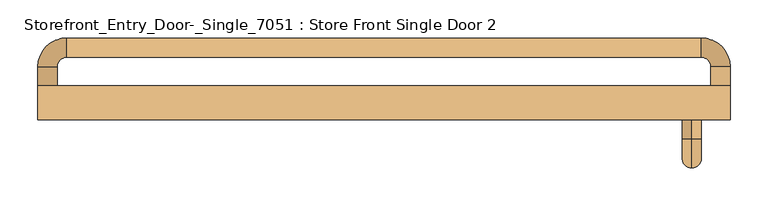
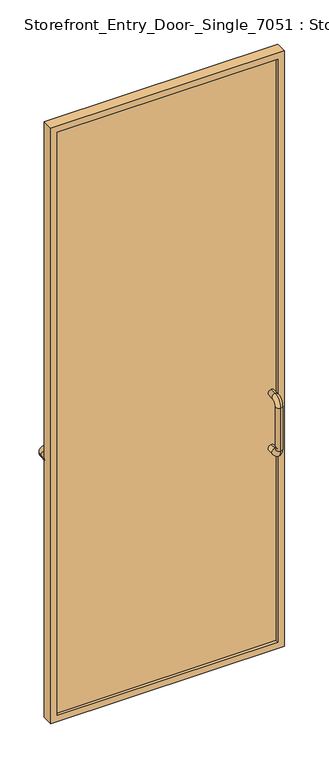
"""IFC4 building model written with IfcOpenShell, lengths in millimetres: door geometry, Storefront_Entry_Door-_Single_7051 : Store Front Single Door 2."""

from ifc_helpers import new_model, si_unit, point, frame, origin, place, context, project, spatial, polyline, circle_curve, ellipse_curve, trimmed, outline, extrude, source, transform, mapped, element, save
from ifc_brep_helpers import plane_surface, cylinder_surface, revolved_surface, advanced_brep


def storefront_entry_door_single_7051_store_front_single_door_2_e2899729(model_context):
    return source(origin(), model_context, "Body", "SolidModel", [
        advanced_brep(
        [(406.4, -25.4, 1054.1), (406.4, -25.4, 1079.5), (406.4, -50.8, 1079.5), (406.4, -50.8, 1054.1), (406.4, -88.9, 1041.4), (406.4, -63.5, 1041.4), (406.4, -88.9, 863.6), (406.4, -63.5, 863.6), (406.4, -50.8, 825.5), (406.4, -50.8, 850.9), (406.4, -25.4, 850.9), (406.4, -25.4, 825.5)],
        [
            (0, 1, circle_curve(frame((406.4, -25.4, 1066.8), z_axis=(0.0, 1.0, 0.0), x_axis=(0.0, 0.0, 1.0)), 12.7)),
            (1, 0, circle_curve(frame((406.4, -25.4, 1066.8), z_axis=(0.0, 1.0, 0.0), x_axis=(0.0, 0.0, 1.0)), 12.7)),
            (1, 2),
            (2, 3, circle_curve(frame((406.4, -50.8, 1066.8), z_axis=(0.0, 1.0, 0.0), x_axis=(0.0, 0.0, 1.0)), 12.7)),
            (3, 0),
            (3, 2, circle_curve(frame((406.4, -50.8, 1066.8), z_axis=(0.0, 1.0, 0.0), x_axis=(0.0, 0.0, 1.0)), 12.7)),
            (4, 5, circle_curve(frame((406.4, -76.2, 1041.4), z_axis=(0.0, 0.0, 1.0), x_axis=(0.0, -1.0, 0.0)), 12.7)),
            (5, 3, circle_curve(frame((406.4, -50.8, 1041.4), z_axis=(-1.0, 0.0, 0.0), x_axis=(0.0, 0.0, 1.0)), 12.7)),
            (2, 4, circle_curve(frame((406.4, -50.8, 1041.4), z_axis=(1.0, 0.0, 0.0), x_axis=(0.0, 0.0, 1.0)), 38.1)),
            (5, 4, circle_curve(frame((406.4, -76.2, 1041.4), z_axis=(0.0, 0.0, 1.0), x_axis=(0.0, -1.0, 0.0)), 12.7)),
            (4, 6),
            (6, 7, circle_curve(frame((406.4, -76.2, 863.6), z_axis=(0.0, 0.0, 1.0), x_axis=(0.0, -1.0, 0.0)), 12.7)),
            (7, 5),
            (7, 6, circle_curve(frame((406.4, -76.2, 863.6), z_axis=(0.0, 0.0, 1.0), x_axis=(0.0, -1.0, 0.0)), 12.7)),
            (8, 9, circle_curve(frame((406.4, -50.8, 838.2), z_axis=(0.0, -1.0, 0.0), x_axis=(0.0, 0.0, -1.0)), 12.7)),
            (9, 7, circle_curve(frame((406.4, -50.8, 863.6), z_axis=(-1.0, 0.0, 0.0), x_axis=(0.0, -1.0, 0.0)), 12.7)),
            (6, 8, circle_curve(frame((406.4, -50.8, 863.6), z_axis=(1.0, 0.0, 0.0), x_axis=(0.0, -1.0, 0.0)), 38.1)),
            (9, 8, circle_curve(frame((406.4, -50.8, 838.2), z_axis=(0.0, -1.0, 0.0), x_axis=(0.0, 0.0, -1.0)), 12.7)),
            (10, 11, circle_curve(frame((406.4, -25.4, 838.2), z_axis=(0.0, 1.0, 0.0), x_axis=(0.0, 0.0, -1.0)), 12.7)),
            (11, 10, circle_curve(frame((406.4, -25.4, 838.2), z_axis=(0.0, 1.0, 0.0), x_axis=(0.0, 0.0, -1.0)), 12.7)),
            (8, 11),
            (10, 9),
        ],
        [
            plane_surface(frame((406.4, -25.4, 1066.8), z_axis=(0.0, 1.0, 0.0), x_axis=(1.0, 0.0, 0.0))),
            cylinder_surface(frame((406.4, -25.4, 1066.8), z_axis=(0.0, 1.0, 0.0), x_axis=(0.0, 0.0, 1.0)), 12.7),
            revolved_surface(trimmed(ellipse_curve(frame((406.4, -50.8, 1066.8), z_axis=(0.0, -1.0, 0.0), x_axis=(0.0, 0.0, 1.0)), 12.7, 12.7), [point((406.4, -50.8, 1054.1))], [point((406.4, -50.8, 1079.5))], True, "CARTESIAN"), (406.4, -50.8, 1041.4), (-1.0, 0.0, 0.0)),
            revolved_surface(trimmed(ellipse_curve(frame((406.4, -50.8, 1066.8), z_axis=(0.0, -1.0, 0.0), x_axis=(0.0, 0.0, 1.0)), 12.7, 12.7), [point((406.4, -50.8, 1079.5))], [point((406.4, -50.8, 1054.1))], True, "CARTESIAN"), (406.4, -50.8, 1041.4), (-1.0, 0.0, 0.0)),
            cylinder_surface(frame((406.4, -76.2, 1041.4), z_axis=(0.0, 0.0, 1.0), x_axis=(0.0, -1.0, 0.0)), 12.7),
            revolved_surface(trimmed(ellipse_curve(frame((406.4, -76.2, 863.6), z_axis=(0.0, 0.0, -1.0), x_axis=(0.0, -1.0, 0.0)), 12.7, 12.7), [point((406.4, -63.5, 863.6))], [point((406.4, -88.9, 863.6))], True, "CARTESIAN"), (406.4, -50.8, 863.6), (-1.0, 0.0, 0.0)),
            revolved_surface(trimmed(ellipse_curve(frame((406.4, -76.2, 863.6), z_axis=(0.0, 0.0, -1.0), x_axis=(0.0, -1.0, 0.0)), 12.7, 12.7), [point((406.4, -88.9, 863.6))], [point((406.4, -63.5, 863.6))], True, "CARTESIAN"), (406.4, -50.8, 863.6), (-1.0, 0.0, 0.0)),
            plane_surface(frame((406.4, -25.4, 838.2), z_axis=(0.0, 1.0, 0.0), x_axis=(1.0, 0.0, 0.0))),
            cylinder_surface(frame((406.4, -50.8, 838.2), z_axis=(0.0, -1.0, 0.0), x_axis=(0.0, 0.0, -1.0)), 12.7),
        ],
        [
            (0, [[1, 2]]),
            (1, [[3, 4, 5, -2]]),
            (1, [[-5, 6, -3, -1]]),
            (2, [[7, 8, -4, 9]]),
            (3, [[10, -9, -6, -8]]),
            (4, [[11, 12, 13, -7]]),
            (4, [[-13, 14, -11, -10]]),
            (5, [[15, 16, -12, 17]]),
            (6, [[18, -17, -14, -16]]),
            (7, [[19, 20]]),
            (8, [[21, -19, 22, -15]]),
            (8, [[-22, -20, -21, -18]]),
        ],
    ),
        advanced_brep(
        [(431.8, 19.05, 1066.8), (457.2, 19.05, 1066.8), (457.2, 44.45, 1066.8), (431.8, 44.45, 1066.8), (419.1, 82.55, 1066.8), (419.1, 57.15, 1066.8), (-419.1, 82.55, 1066.8), (-419.1, 57.15, 1066.8), (-457.2, 44.45, 1066.8), (-431.8, 44.45, 1066.8), (-431.8, 19.05, 1066.8), (-457.2, 19.05, 1066.8)],
        [
            (0, 1, circle_curve(frame((444.5, 19.05, 1066.8), z_axis=(0.0, -1.0, 0.0), x_axis=(1.0, 0.0, 0.0)), 12.7)),
            (1, 0, circle_curve(frame((444.5, 19.05, 1066.8), z_axis=(0.0, -1.0, 0.0), x_axis=(1.0, 0.0, 0.0)), 12.7)),
            (1, 2),
            (2, 3, circle_curve(frame((444.5, 44.45, 1066.8), z_axis=(0.0, -1.0, 0.0), x_axis=(1.0, 0.0, 0.0)), 12.7)),
            (3, 0),
            (3, 2, circle_curve(frame((444.5, 44.45, 1066.8), z_axis=(0.0, -1.0, 0.0), x_axis=(1.0, 0.0, 0.0)), 12.7)),
            (4, 5, circle_curve(frame((419.1, 69.85, 1066.8), z_axis=(1.0, 0.0, 0.0), x_axis=(0.0, 1.0, 0.0)), 12.7)),
            (5, 3, circle_curve(frame((419.1, 44.45, 1066.8), z_axis=(0.0, 0.0, -1.0), x_axis=(1.0, 0.0, 0.0)), 12.7)),
            (2, 4, circle_curve(frame((419.1, 44.45, 1066.8), z_axis=(0.0, 0.0, 1.0), x_axis=(1.0, 0.0, 0.0)), 38.1)),
            (5, 4, circle_curve(frame((419.1, 69.85, 1066.8), z_axis=(1.0, 0.0, 0.0), x_axis=(0.0, 1.0, 0.0)), 12.7)),
            (4, 6),
            (6, 7, circle_curve(frame((-419.1, 69.85, 1066.8), z_axis=(1.0, 0.0, 0.0), x_axis=(0.0, 1.0, 0.0)), 12.7)),
            (7, 5),
            (7, 6, circle_curve(frame((-419.1, 69.85, 1066.8), z_axis=(1.0, 0.0, 0.0), x_axis=(0.0, 1.0, 0.0)), 12.7)),
            (8, 9, circle_curve(frame((-444.5, 44.45, 1066.8), z_axis=(0.0, 1.0, 0.0), x_axis=(-1.0, 0.0, 0.0)), 12.7)),
            (9, 7, circle_curve(frame((-419.1, 44.45, 1066.8), z_axis=(0.0, 0.0, -1.0), x_axis=(0.0, 1.0, 0.0)), 12.7)),
            (6, 8, circle_curve(frame((-419.1, 44.45, 1066.8), z_axis=(0.0, 0.0, 1.0), x_axis=(0.0, 1.0, 0.0)), 38.1)),
            (9, 8, circle_curve(frame((-444.5, 44.45, 1066.8), z_axis=(0.0, 1.0, 0.0), x_axis=(-1.0, 0.0, 0.0)), 12.7)),
            (10, 11, circle_curve(frame((-444.5, 19.05, 1066.8), z_axis=(0.0, -1.0, 0.0), x_axis=(-1.0, 0.0, 0.0)), 12.7)),
            (11, 10, circle_curve(frame((-444.5, 19.05, 1066.8), z_axis=(0.0, -1.0, 0.0), x_axis=(-1.0, 0.0, 0.0)), 12.7)),
            (8, 11),
            (10, 9),
        ],
        [
            plane_surface(frame((444.5, 19.05, 1066.8), z_axis=(0.0, -1.0, 0.0), x_axis=(0.0, 0.0, 1.0))),
            cylinder_surface(frame((444.5, 19.05, 1066.8), z_axis=(0.0, -1.0, 0.0), x_axis=(1.0, 0.0, 0.0)), 12.7),
            revolved_surface(trimmed(ellipse_curve(frame((444.5, 44.45, 1066.8), z_axis=(0.0, 1.0, 0.0), x_axis=(1.0, 0.0, 0.0)), 12.7, 12.7), [point((431.8, 44.45, 1066.8))], [point((457.2, 44.45, 1066.8))], True, "CARTESIAN"), (419.1, 44.45, 1066.8), (0.0, 0.0, -1.0)),
            revolved_surface(trimmed(ellipse_curve(frame((444.5, 44.45, 1066.8), z_axis=(0.0, 1.0, 0.0), x_axis=(1.0, 0.0, 0.0)), 12.7, 12.7), [point((457.2, 44.45, 1066.8))], [point((431.8, 44.45, 1066.8))], True, "CARTESIAN"), (419.1, 44.45, 1066.8), (0.0, 0.0, -1.0)),
            cylinder_surface(frame((419.1, 69.85, 1066.8), z_axis=(1.0, 0.0, 0.0), x_axis=(0.0, 1.0, 0.0)), 12.7),
            revolved_surface(trimmed(ellipse_curve(frame((-419.1, 69.85, 1066.8), z_axis=(-1.0, 0.0, 0.0), x_axis=(0.0, 1.0, 0.0)), 12.7, 12.7), [point((-419.1, 57.15, 1066.8))], [point((-419.1, 82.55, 1066.8))], True, "CARTESIAN"), (-419.1, 44.45, 1066.8), (0.0, 0.0, -1.0)),
            revolved_surface(trimmed(ellipse_curve(frame((-419.1, 69.85, 1066.8), z_axis=(-1.0, 0.0, 0.0), x_axis=(0.0, 1.0, 0.0)), 12.7, 12.7), [point((-419.1, 82.55, 1066.8))], [point((-419.1, 57.15, 1066.8))], True, "CARTESIAN"), (-419.1, 44.45, 1066.8), (0.0, 0.0, -1.0)),
            plane_surface(frame((-444.5, 19.05, 1066.8), z_axis=(0.0, -1.0, 0.0), x_axis=(0.0, 0.0, 1.0))),
            cylinder_surface(frame((-444.5, 44.45, 1066.8), z_axis=(0.0, 1.0, 0.0), x_axis=(-1.0, 0.0, 0.0)), 12.7),
        ],
        [
            (0, [[1, 2]]),
            (1, [[3, 4, 5, -2]]),
            (1, [[-5, 6, -3, -1]]),
            (2, [[7, 8, -4, 9]]),
            (3, [[10, -9, -6, -8]]),
            (4, [[11, 12, 13, -7]]),
            (4, [[-13, 14, -11, -10]]),
            (5, [[15, 16, -12, 17]]),
            (6, [[18, -17, -14, -16]]),
            (7, [[19, 20]]),
            (8, [[21, -19, 22, -15]]),
            (8, [[-22, -20, -21, -18]]),
        ],
    ),
        extrude(outline(polyline([(431.8, 6.35), (431.8, -12.7), (-431.8, -12.7), (-431.8, 6.35), (431.8, 6.35)])), frame((0.0, 0.0, 25.4), z_axis=(0.0, 0.0, 1.0), x_axis=(1.0, 0.0, 0.0)), (0.0, 0.0, 1.0), 2409.825),
        extrude(outline(polyline([(2460.625, 457.2), (2460.625, -457.2), (0.0, -457.2), (0.0, 457.2), (2460.625, 457.2)]), holes=[polyline([(2435.225, -431.8), (2435.225, 431.8), (25.4, 431.8), (25.4, -431.8), (2435.225, -431.8)])]), frame((0.0, -25.4, 0.0), z_axis=(0.0, 1.0, 0.0), x_axis=(0.0, 0.0, 1.0)), (0.0, 0.0, 1.0), 44.45),
    ])


if __name__ == "__main__":
    model = new_model("IFC4")
    model_context = context("Model", 3, world=origin())
    ifc_project = project(units=[si_unit("LENGTHUNIT", "METRE", prefix="MILLI")], contexts=[model_context])
    site = spatial("IfcSite", under=ifc_project)
    building = spatial("IfcBuilding", under=site)
    placement = place(None, origin())
    storefront_entry_door_single_7051_store_front_single_door_2_shape = storefront_entry_door_single_7051_store_front_single_door_2_e2899729(model_context)
    element("IfcDoor", 1, ObjectType="Storefront_Entry_Door-_Single_7051 : Store Front Single Door 2", at=placement, inside=building, context=model_context, shape_type="MappedRepresentation", body=[
        mapped(storefront_entry_door_single_7051_store_front_single_door_2_shape, transform((0.0, 0.0, 0.0), x_axis=(1.0, 0.0, 0.0), y_axis=(0.0, 1.0, 0.0), z_axis=(0.0, 0.0, 1.0))),
    ])
    save(model, "model.ifc")

# Revit data of these elements
# Type "Storefront_Entry_Door-_Single_7051 : Store Front Single Door 2"
#   Type Mark = "31"
#   Assembly Code = "B2030110"
#   Analytic Construction = "<None>"
#   Top Rail = 0' - 1"
#   Side Rail = 0' - 1"
#   Reporting Width [instance default] = 4' - 2"
#   Rail Height AFF = 3' - 6"
#   Offset = 0' - 1"
#   Door Width [instance default] = 4' - 2"
#   Bottom Rail Width = 0' - 1"
#   Material = Metal - Aluminum
#   Glazing Material = Glass
#   Function = (empty or 0)
# Element 1 (IfcDoor, "Storefront_Entry_Door-_Single_7051 : Store Front Single Door 2")
#   Reporting Width = 3' - 0"
#   Door Width = 3' - 0"
#   Materials on its faces: "Metal - Aluminum", "Glass"
# Materials
#   "Metal - Aluminum": class "Metal", colour RGB 247 247 247, transparency 0
#   "Glass": class "Glass", colour RGB 218 227 224, transparency 0.85, Description = "Soda Lime Glass", Cost = 0
